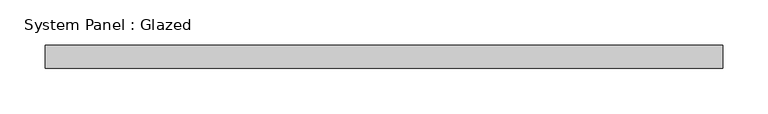
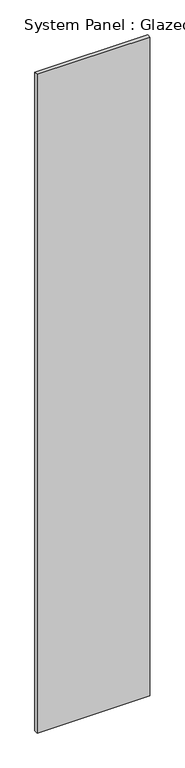
"""IFC4 building model written with IfcOpenShell, lengths in millimetres: plate geometry, System Panel : Glazed."""

import ifcopenshell
import ifcopenshell.guid

model = None  # the IFC model being written
_history = None  # IfcOwnerHistory: only IFC2X3 demands one
_inside = {}  # id of a spatial element -> (the spatial element, [elements in it])
_under = {}  # id of a project, library or spatial element -> (it, [spatial elements below it])
_declared = {}  # id of a project -> (the project, [libraries it declares])
_typed = {}  # id of a type object -> (the type object, [elements of that type])
_made_of = {}  # id of a material, layer set ... -> (it, [elements and type objects made of it])


def new_model(schema):
    """Start an empty IFC model of exactly this schema.

    Asked for "IFC4X3", IfcOpenShell would pick the latest addendum, in which some entities
    have other attributes; the version numbers below select the first issue.
    IFC2X3 requires an IfcOwnerHistory on every rooted entity: one is made here for all.
    """
    global model, _history
    if schema == "IFC4X3":
        model = ifcopenshell.file(schema_version=(4, 3, 0, 0))
    else:
        model = ifcopenshell.file(schema=schema)
    _inside.clear()
    _under.clear()
    _declared.clear()
    _typed.clear()
    _made_of.clear()
    _history = None
    if model.schema == "IFC2X3":
        org = make("IfcOrganization", Name="unknown")
        user = make(
            "IfcPersonAndOrganization",
            ThePerson=make("IfcPerson", FamilyName="unknown"),
            TheOrganization=org,
        )
        app = make(
            "IfcApplication",
            ApplicationDeveloper=org,
            Version="unknown",
            ApplicationFullName="unknown",
            ApplicationIdentifier="unknown",
        )
        _history = make(
            "IfcOwnerHistory",
            OwningUser=user,
            OwningApplication=app,
            ChangeAction="ADDED",
            CreationDate=0,
        )
    return model


def make(cls, **values):
    """One entity of the class cls with the attributes given. An attribute that is None is left unset."""
    return model.create_entity(
        cls, **{name: value for name, value in values.items() if value is not None}
    )


def rooted(cls, **values):
    """An entity with a GlobalId (a new one), such as an element, a storey or a relation."""
    return make(cls, GlobalId=ifcopenshell.guid.new(), OwnerHistory=_history, **values)


def si_unit(unit_type, name, prefix=None):
    """IfcSIUnit, for example si_unit("LENGTHUNIT", "METRE", prefix="MILLI")."""
    return make("IfcSIUnit", UnitType=unit_type, Prefix=prefix, Name=name)


def assignment(units):
    """IfcUnitAssignment: the units of a project."""
    return None if units is None else make("IfcUnitAssignment", Units=units)


def point(xyz):
    """IfcCartesianPoint."""
    return None if xyz is None else make("IfcCartesianPoint", Coordinates=xyz)


def direction(xyz):
    """IfcDirection."""
    return None if xyz is None else make("IfcDirection", DirectionRatios=xyz)


def frame(location, z_axis=None, x_axis=None):
    """IfcAxis2Placement3D, a coordinate frame: its origin and axes. An axis left out is left unset."""
    return make(
        "IfcAxis2Placement3D",
        Location=point(location),
        Axis=direction(z_axis),
        RefDirection=direction(x_axis),
    )


def origin():
    """The frame at (0, 0, 0) with its axes left unset."""
    return frame((0.0, 0.0, 0.0))


def origin_with_axes():
    """The frame at (0, 0, 0) with the z axis (0, 0, 1) and the x axis (1, 0, 0) written out."""
    return frame((0.0, 0.0, 0.0), z_axis=(0.0, 0.0, 1.0), x_axis=(1.0, 0.0, 0.0))


def place(relative_to, where):
    """IfcLocalPlacement: puts the frame where relative to a parent placement (None: the world)."""
    return make(
        "IfcLocalPlacement", PlacementRelTo=relative_to, RelativePlacement=where
    )


def context(
    kind, dimensions, precision=None, world=None, true_north=None, identifier=None
):
    """IfcGeometricRepresentationContext, for example the 3D "Model" context."""
    return make(
        "IfcGeometricRepresentationContext",
        ContextIdentifier=identifier,
        ContextType=kind,
        CoordinateSpaceDimension=dimensions,
        Precision=precision,
        WorldCoordinateSystem=world,
        TrueNorth=true_north,
    )


def project(units=None, contexts=None):
    """IfcProject with its units and contexts."""
    return rooted(
        "IfcProject",
        Name="project",
        RepresentationContexts=contexts,
        UnitsInContext=assignment(units),
    )


def spatial(cls, under=None, at=None, **own):
    """A site, building, storey or space (cls), placed at a placement, below another one or the project."""
    s = rooted(cls, ObjectPlacement=at, **own)
    if under is not None:
        _under.setdefault(under.id(), (under, []))[1].append(s)
    return s


def polyline(points):
    """IfcPolyline through the points."""
    return make("IfcPolyline", Points=[point(p) for p in points])


def outline(outer, holes=None, kind="AREA"):
    """IfcArbitraryClosedProfileDef: a profile drawn as a closed curve; with holes, ...WithVoids."""
    if holes is None:
        return make("IfcArbitraryClosedProfileDef", ProfileType=kind, OuterCurve=outer)
    return make(
        "IfcArbitraryProfileDefWithVoids",
        ProfileType=kind,
        OuterCurve=outer,
        InnerCurves=holes,
    )


def extrude(swept, where, along, depth):
    """IfcExtrudedAreaSolid: the profile swept, set in the frame where, extruded along a direction by depth."""
    return make(
        "IfcExtrudedAreaSolid",
        SweptArea=swept,
        Position=where,
        ExtrudedDirection=direction(along),
        Depth=depth,
    )


def shape(context_of_items, identifier, shape_type, items):
    """IfcShapeRepresentation: the items that make up one representation, for example the "Body"."""
    return make(
        "IfcShapeRepresentation",
        ContextOfItems=context_of_items,
        RepresentationIdentifier=identifier,
        RepresentationType=shape_type,
        Items=items,
    )


def source(mapping_origin, context_of_items, identifier, shape_type, items):
    """IfcRepresentationMap: a shape defined once, which mapped items show again and again."""
    return make(
        "IfcRepresentationMap",
        MappingOrigin=mapping_origin,
        MappedRepresentation=shape(context_of_items, identifier, shape_type, items),
    )


def transform(
    local_origin,
    x_axis=None,
    y_axis=None,
    z_axis=None,
    scale=None,
    scale2=None,
    scale3=None,
    uniform=True,
):
    """IfcCartesianTransformationOperator3D, or its non-uniform kind. x_axis, y_axis, z_axis: its Axis1, 2, 3."""
    if uniform:
        return make(
            "IfcCartesianTransformationOperator3D",
            Axis1=direction(x_axis),
            Axis2=direction(y_axis),
            LocalOrigin=point(local_origin),
            Scale=scale,
            Axis3=direction(z_axis),
        )
    return make(
        "IfcCartesianTransformationOperator3DnonUniform",
        Axis1=direction(x_axis),
        Axis2=direction(y_axis),
        LocalOrigin=point(local_origin),
        Scale=scale,
        Axis3=direction(z_axis),
        Scale2=scale2,
        Scale3=scale3,
    )


def mapped(mapping_source, mapping_target):
    """IfcMappedItem: shows the shape of a source again, moved by a transform."""
    return make(
        "IfcMappedItem", MappingSource=mapping_source, MappingTarget=mapping_target
    )


def made_of(thing, what):
    """Note that an element or type object is made of a material, layer set ...; save() writes the relation."""
    if what is not None:
        _made_of.setdefault(what.id(), (what, []))[1].append(thing)
    return thing


def element(
    cls,
    number,
    at=None,
    inside=None,
    cuts=None,
    type_object=None,
    material=None,
    context=None,
    identifier="Body",
    shape_type=None,
    held_by="IfcProductDefinitionShape",
    body=None,
    shapes=None,
    **own,
):
    """One element of the class cls, such as IfcWall. Its Tag is "e" and its number.

    at: its placement. inside: the storey or other place that contains it. cuts: it is an
    opening in that element (IfcRelVoidsElement). A single representation is given by context,
    identifier, shape_type and body (its items); several are given by shapes. held_by: the class
    of the entity that holds the representations. save() writes the other relations.
    """
    e = rooted(cls, Tag="e%d" % number, ObjectPlacement=at, **own)
    if body is not None:
        shapes = [shape(context, identifier, shape_type, body)]
    if shapes is not None:
        e.Representation = make(held_by, Representations=shapes)
    if inside is not None:
        _inside.setdefault(inside.id(), (inside, []))[1].append(e)
    if cuts is not None:
        rooted(
            "IfcRelVoidsElement", RelatingBuildingElement=cuts, RelatedOpeningElement=e
        )
    if type_object is not None:
        _typed.setdefault(type_object.id(), (type_object, []))[1].append(e)
    return made_of(e, material)


def aggregate(whole, parts):
    """IfcRelAggregates: a whole, such as a stair, and the parts it consists of."""
    return rooted("IfcRelAggregates", RelatingObject=whole, RelatedObjects=parts)


def save(model, path):
    """Write the relations noted so far, then the file.

    IfcRelAggregates (storeys below a building ...), IfcRelContainedInSpatialStructure (elements
    in a storey), IfcRelDefinesByType, IfcRelAssociatesMaterial and IfcRelDeclares: one each for
    every whole, place, type object, material and project.
    """
    for whole, parts in _under.values():
        aggregate(whole, parts)
    for where, things in _inside.values():
        rooted(
            "IfcRelContainedInSpatialStructure",
            RelatedElements=things,
            RelatingStructure=where,
        )
    for kind, things in _typed.values():
        rooted("IfcRelDefinesByType", RelatedObjects=things, RelatingType=kind)
    for what, things in _made_of.values():
        rooted("IfcRelAssociatesMaterial", RelatedObjects=things, RelatingMaterial=what)
    for by, libraries in _declared.values():
        rooted("IfcRelDeclares", RelatingContext=by, RelatedDefinitions=libraries)
    model.write(path)


def system_panel_glazed_ccbaed92(model_context):
    return source(origin(), model_context, "Body", "SweptSolid", [
        extrude(outline(polyline([(375.1494819, 19.05), (-375.1494819, 19.05), (-375.1494819, 44.45), (375.1494819, 44.45), (375.1494819, 19.05)])), origin_with_axes(), (0.0, 0.0, 1.0), 4629.15),
    ])


if __name__ == "__main__":
    model = new_model("IFC4")
    model_context = context("Model", 3, world=origin())
    ifc_project = project(units=[si_unit("LENGTHUNIT", "METRE", prefix="MILLI")], contexts=[model_context])
    site = spatial("IfcSite", under=ifc_project)
    building = spatial("IfcBuilding", under=site)
    placement = place(None, origin())
    system_panel_glazed_shape = system_panel_glazed_ccbaed92(model_context)
    element("IfcPlate", 1, ObjectType="System Panel : Glazed", at=placement, inside=building, context=model_context, shape_type="MappedRepresentation", body=[
        mapped(system_panel_glazed_shape, transform((0.0, 0.0, 0.0), x_axis=(1.0, 0.0, 0.0), y_axis=(0.0, 1.0, 0.0), z_axis=(0.0, 0.0, 1.0))),
    ])
    save(model, "model.ifc")

# Revit data of these elements
# Type "System Panel : Glazed"
#   Construction Type Id = "GSP4R"
#   Analytic Construction = "1/8 in Pilkington single glazing"
#   Visual Light Transmittance = 0.9
#   Solar Heat Gain Coefficient = 0.86
#   Heat Transfer Coefficient (U) = 1.18115 BTU/(h·ft²·°F)
#   Define Thermal Properties by = 1
# Element 1 (IfcPlate, "System Panel : Glazed")
#   Materials on its faces: "Glass"
# Materials
#   "Glass": class "Glass", colour RGB 0 128 192, transparency 0.75, Description = "Soda Lime Glass", Cost = 0
